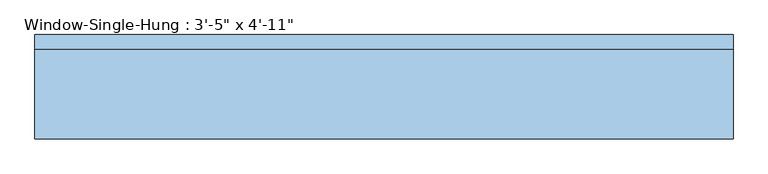
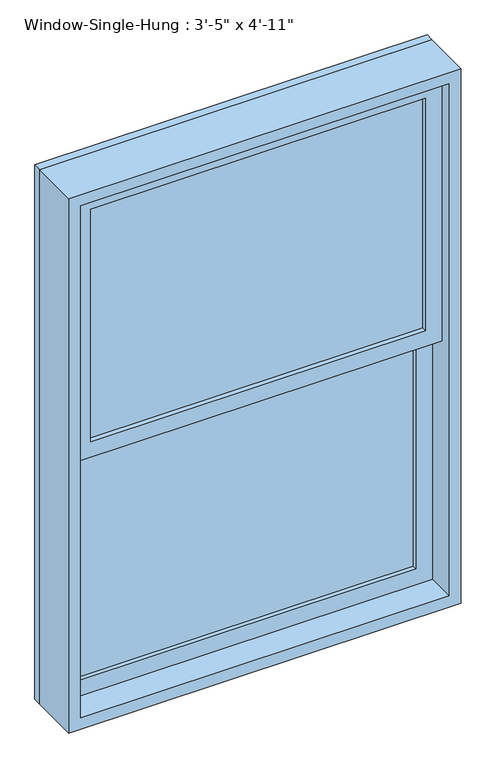
"""IFC4 building model written with IfcOpenShell, lengths in millimetres: window geometry."""

from ifc_helpers import new_model, si_unit, frame, origin, place, context, project, spatial, polyline, outline, extrude, source, transform, mapped, element, save


def window_d73c3647(model_context):
    return source(origin(), model_context, "Body", "SweptSolid", [
        extrude(outline(polyline([(444.5, 1.5875), (-444.5, 1.5875), (-444.5, 7.9375), (444.5, 7.9375), (444.5, 1.5875)])), frame((0.0, 0.0, 990.6), z_axis=(0.0, 0.0, 1.0), x_axis=(1.0, 0.0, 0.0)), (0.0, 0.0, 1.0), 650.875),
        extrude(outline(polyline([(-444.5, 14.2875), (-444.5, 20.6375), (444.5, 20.6375), (444.5, 14.2875), (-444.5, 14.2875)])), frame((0.0, 0.0, 990.6), z_axis=(0.0, 0.0, 1.0), x_axis=(1.0, 0.0, 0.0)), (0.0, 0.0, 1.0), 650.875),
        extrude(outline(polyline([(444.5, -42.8625), (-444.5, -42.8625), (-444.5, -36.5125), (444.5, -36.5125), (444.5, -42.8625)])), frame((0.0, 0.0, 1685.925), z_axis=(0.0, 0.0, 1.0), x_axis=(1.0, 0.0, 0.0)), (0.0, 0.0, 1.0), 650.875),
        extrude(outline(polyline([(-444.5, -30.1625), (-444.5, -23.8125), (444.5, -23.8125), (444.5, -30.1625), (-444.5, -30.1625)])), frame((0.0, 0.0, 1685.925), z_axis=(0.0, 0.0, 1.0), x_axis=(1.0, 0.0, 0.0)), (0.0, 0.0, 1.0), 650.875),
        extrude(outline(polyline([(1685.925, 488.95), (1685.925, -488.95), (946.15, -488.95), (946.15, 488.95), (1685.925, 488.95)]), holes=[polyline([(1641.475, -444.5), (1641.475, 444.5), (990.6, 444.5), (990.6, -444.5), (1641.475, -444.5)])]), frame((0.0, -11.1125, 0.0), z_axis=(0.0, 1.0, 0.0), x_axis=(0.0, 0.0, 1.0)), (0.0, 0.0, 1.0), 44.45),
        extrude(outline(polyline([(2381.25, 488.95), (2381.25, -488.95), (1641.475, -488.95), (1641.475, 488.95), (2381.25, 488.95)]), holes=[polyline([(2336.8, -444.5), (2336.8, 444.5), (1685.925, 444.5), (1685.925, -444.5), (2336.8, -444.5)])]), frame((0.0, -55.5625, 0.0), z_axis=(0.0, 1.0, 0.0), x_axis=(0.0, 0.0, 1.0)), (0.0, 0.0, 1.0), 44.45),
        extrude(outline(polyline([(2413.0, 520.7), (2413.0, -520.7), (914.4, -520.7), (914.4, 520.7), (2413.0, 520.7)]), holes=[polyline([(2381.25, -488.95), (2381.25, 488.95), (946.15, 488.95), (946.15, -488.95), (2381.25, -488.95)])]), frame((0.0, -87.3125, 0.0), z_axis=(0.0, 1.0, 0.0), x_axis=(0.0, 0.0, 1.0)), (0.0, 0.0, 1.0), 133.35),
        extrude(outline(polyline([(2413.0, 520.7), (2413.0, -520.7), (914.4, -520.7), (914.4, 520.7), (2413.0, 520.7)]), holes=[polyline([(2393.95, 501.65), (933.45, 501.65), (933.45, -501.65), (2393.95, -501.65), (2393.95, 501.65)])]), frame((0.0, 46.0375, 0.0), z_axis=(0.0, 1.0, 0.0), x_axis=(0.0, 0.0, 1.0)), (0.0, 0.0, 1.0), 22.225),
    ])


if __name__ == "__main__":
    model = new_model("IFC4")
    model_context = context("Model", 3, world=origin())
    ifc_project = project(units=[si_unit("LENGTHUNIT", "METRE", prefix="MILLI")], contexts=[model_context])
    site = spatial("IfcSite", under=ifc_project)
    building = spatial("IfcBuilding", under=site)
    placement = place(None, origin())
    window_shape = window_d73c3647(model_context)
    element("IfcWindow", 1, ObjectType="Window-Single-Hung : 3'-5\" x 4'-11\"", at=placement, inside=building, context=model_context, shape_type="MappedRepresentation", body=[
        mapped(window_shape, transform((0.0, 0.0, 0.0), x_axis=(1.0, 0.0, 0.0), y_axis=(0.0, 1.0, 0.0), z_axis=(0.0, 0.0, 1.0))),
    ])
    save(model, "model.ifc")

# Revit data of these elements
# Type "Window-Single-Hung : 3'-5\" x 4'-11\""
#   Type Mark = "21"
#   Fire Rating = "0.5h"
#   Construction Type Id = "DG-DR"
#   Assembly Code = "B2020100"
#   Analytic Construction = "Double glazing - domestic"
#   Wall Thickness [instance default] = 0' - 6"
#   Window Inset [instance default] = 0' - 0"
#   Visual Light Transmittance = 0.81
#   Thermal Resistance (R) = 0.319569 (m²·K)/W
#   Solar Heat Gain Coefficient = 0.76
#   Muntin Width = 2' - 11"
#   Muntin Height = 2' - 1 5/8"
#   Interior Wall Closure [instance default] = 0' - 1 1/2"
#   Rough Width = 3' - 5 1/2"
#   Rough Height = 4' - 11 1/2"
#   Frame Extension [instance default] = 0' - 1 1/4"
#   Exterior Wall Closure [instance default] = 0' - 0 1/2"
#   Extension Jamb [instance default] = 0' - 1 1/2"
#   Heat Transfer Coefficient (U) = 3.12929 W/(m²·K)
#   Height = 4' - 11"
#   Width = 3' - 5"
#   Top Muntin Visibility = yes
#   Indicator Visibility [instance default] = yes
#   Extension Jamb Visibility [instance default] = yes
#   Interior Trim Visibility [instance default] = yes
#   Exterior Trim Visibility [instance default] = yes
#   Bottom Muntin Visibility = yes
#   Muntin Pattern = Muntin Pattern_2x2 : Muntin Pattern_2x2
#   Interior Trim Material = Wood - Stained
#   Interior Trim = Trim-Window-Interior-Flat : Picture Frame
#   Exterior Trim Material = Clad - White
#   Exterior Trim = Trim-Window-Exterior-Flat : with Sill
#   Glass Panel Material = Glass
#   Exterior Frame Material = Clad - White
#   Interior Frame Material = Wood - Stained
#   Wall Closure = (empty or 0)
# Element 1 (IfcWindow, "Window-Single-Hung : 3'-5\" x 4'-11\"")
#   Wall Thickness = 0' - 5 3/8"
#   Extension Jamb = 0' - 0 7/8"
#   Materials on its faces: "Wood - Stained", "Glass", "Clad - White"
# Materials
#   "Wood - Stained": class "Wood", colour RGB 224 178 126, transparency 0, Cost = 0
#   "Clad - White": class "Wood", colour RGB 242 242 238, transparency 0, Cost = 0
#   "Glass": class "Glass", colour RGB 0 128 192, transparency 0.75, Description = "Soda Lime Glass", Cost = 0
